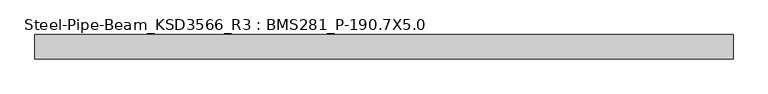
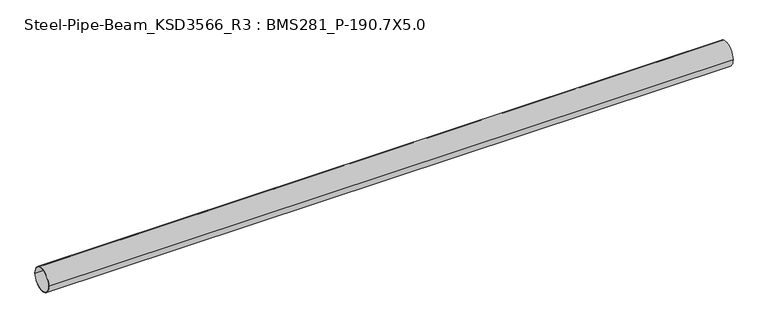
"""IFC4 building model written with IfcOpenShell, lengths in millimetres: member geometry, Steel-Pipe-Beam_KSD3566_R3 : BMS281_P-190.7X5.0."""

import ifcopenshell
import ifcopenshell.guid

model = None  # the IFC model being written
_history = None  # IfcOwnerHistory: only IFC2X3 demands one
_inside = {}  # id of a spatial element -> (the spatial element, [elements in it])
_under = {}  # id of a project, library or spatial element -> (it, [spatial elements below it])
_declared = {}  # id of a project -> (the project, [libraries it declares])
_typed = {}  # id of a type object -> (the type object, [elements of that type])
_made_of = {}  # id of a material, layer set ... -> (it, [elements and type objects made of it])


def new_model(schema):
    """Start an empty IFC model of exactly this schema.

    Asked for "IFC4X3", IfcOpenShell would pick the latest addendum, in which some entities
    have other attributes; the version numbers below select the first issue.
    IFC2X3 requires an IfcOwnerHistory on every rooted entity: one is made here for all.
    """
    global model, _history
    if schema == "IFC4X3":
        model = ifcopenshell.file(schema_version=(4, 3, 0, 0))
    else:
        model = ifcopenshell.file(schema=schema)
    _inside.clear()
    _under.clear()
    _declared.clear()
    _typed.clear()
    _made_of.clear()
    _history = None
    if model.schema == "IFC2X3":
        org = make("IfcOrganization", Name="unknown")
        user = make(
            "IfcPersonAndOrganization",
            ThePerson=make("IfcPerson", FamilyName="unknown"),
            TheOrganization=org,
        )
        app = make(
            "IfcApplication",
            ApplicationDeveloper=org,
            Version="unknown",
            ApplicationFullName="unknown",
            ApplicationIdentifier="unknown",
        )
        _history = make(
            "IfcOwnerHistory",
            OwningUser=user,
            OwningApplication=app,
            ChangeAction="ADDED",
            CreationDate=0,
        )
    return model


def make(cls, **values):
    """One entity of the class cls with the attributes given. An attribute that is None is left unset."""
    return model.create_entity(
        cls, **{name: value for name, value in values.items() if value is not None}
    )


def rooted(cls, **values):
    """An entity with a GlobalId (a new one), such as an element, a storey or a relation."""
    return make(cls, GlobalId=ifcopenshell.guid.new(), OwnerHistory=_history, **values)


def si_unit(unit_type, name, prefix=None):
    """IfcSIUnit, for example si_unit("LENGTHUNIT", "METRE", prefix="MILLI")."""
    return make("IfcSIUnit", UnitType=unit_type, Prefix=prefix, Name=name)


def assignment(units):
    """IfcUnitAssignment: the units of a project."""
    return None if units is None else make("IfcUnitAssignment", Units=units)


def point(xyz):
    """IfcCartesianPoint."""
    return None if xyz is None else make("IfcCartesianPoint", Coordinates=xyz)


def direction(xyz):
    """IfcDirection."""
    return None if xyz is None else make("IfcDirection", DirectionRatios=xyz)


def frame(location, z_axis=None, x_axis=None):
    """IfcAxis2Placement3D, a coordinate frame: its origin and axes. An axis left out is left unset."""
    return make(
        "IfcAxis2Placement3D",
        Location=point(location),
        Axis=direction(z_axis),
        RefDirection=direction(x_axis),
    )


def frame_2d(location, x_axis=None):
    """IfcAxis2Placement2D, a coordinate frame in the plane: its origin and x axis."""
    return make(
        "IfcAxis2Placement2D", Location=point(location), RefDirection=direction(x_axis)
    )


def origin():
    """The frame at (0, 0, 0) with its axes left unset."""
    return frame((0.0, 0.0, 0.0))


def origin_2d():
    """The frame at (0, 0) in the plane with its x axis left unset."""
    return frame_2d((0.0, 0.0))


def place(relative_to, where):
    """IfcLocalPlacement: puts the frame where relative to a parent placement (None: the world)."""
    return make(
        "IfcLocalPlacement", PlacementRelTo=relative_to, RelativePlacement=where
    )


def context(
    kind, dimensions, precision=None, world=None, true_north=None, identifier=None
):
    """IfcGeometricRepresentationContext, for example the 3D "Model" context."""
    return make(
        "IfcGeometricRepresentationContext",
        ContextIdentifier=identifier,
        ContextType=kind,
        CoordinateSpaceDimension=dimensions,
        Precision=precision,
        WorldCoordinateSystem=world,
        TrueNorth=true_north,
    )


def project(units=None, contexts=None):
    """IfcProject with its units and contexts."""
    return rooted(
        "IfcProject",
        Name="project",
        RepresentationContexts=contexts,
        UnitsInContext=assignment(units),
    )


def spatial(cls, under=None, at=None, **own):
    """A site, building, storey or space (cls), placed at a placement, below another one or the project."""
    s = rooted(cls, ObjectPlacement=at, **own)
    if under is not None:
        _under.setdefault(under.id(), (under, []))[1].append(s)
    return s


def circle_curve(where, radius):
    """IfcCircle in the frame where."""
    return make("IfcCircle", Position=where, Radius=radius)


def trimmed(basis, trim1, trim2, sense, master):
    """IfcTrimmedCurve: the piece of a basis curve between two trims."""
    return make(
        "IfcTrimmedCurve",
        BasisCurve=basis,
        Trim1=trim1,
        Trim2=trim2,
        SenseAgreement=sense,
        MasterRepresentation=master,
    )


def segment(curve, same_sense, transition):
    """IfcCompositeCurveSegment."""
    return make(
        "IfcCompositeCurveSegment",
        Transition=transition,
        SameSense=same_sense,
        ParentCurve=curve,
    )


def composite_curve(segments, self_intersect=None):
    """IfcCompositeCurve: segments joined end to end."""
    return make("IfcCompositeCurve", Segments=segments, SelfIntersect=self_intersect)


def outline(outer, holes=None, kind="AREA"):
    """IfcArbitraryClosedProfileDef: a profile drawn as a closed curve; with holes, ...WithVoids."""
    if holes is None:
        return make("IfcArbitraryClosedProfileDef", ProfileType=kind, OuterCurve=outer)
    return make(
        "IfcArbitraryProfileDefWithVoids",
        ProfileType=kind,
        OuterCurve=outer,
        InnerCurves=holes,
    )


def extrude(swept, where, along, depth):
    """IfcExtrudedAreaSolid: the profile swept, set in the frame where, extruded along a direction by depth."""
    return make(
        "IfcExtrudedAreaSolid",
        SweptArea=swept,
        Position=where,
        ExtrudedDirection=direction(along),
        Depth=depth,
    )


def shape(context_of_items, identifier, shape_type, items):
    """IfcShapeRepresentation: the items that make up one representation, for example the "Body"."""
    return make(
        "IfcShapeRepresentation",
        ContextOfItems=context_of_items,
        RepresentationIdentifier=identifier,
        RepresentationType=shape_type,
        Items=items,
    )


def source(mapping_origin, context_of_items, identifier, shape_type, items):
    """IfcRepresentationMap: a shape defined once, which mapped items show again and again."""
    return make(
        "IfcRepresentationMap",
        MappingOrigin=mapping_origin,
        MappedRepresentation=shape(context_of_items, identifier, shape_type, items),
    )


def transform(
    local_origin,
    x_axis=None,
    y_axis=None,
    z_axis=None,
    scale=None,
    scale2=None,
    scale3=None,
    uniform=True,
):
    """IfcCartesianTransformationOperator3D, or its non-uniform kind. x_axis, y_axis, z_axis: its Axis1, 2, 3."""
    if uniform:
        return make(
            "IfcCartesianTransformationOperator3D",
            Axis1=direction(x_axis),
            Axis2=direction(y_axis),
            LocalOrigin=point(local_origin),
            Scale=scale,
            Axis3=direction(z_axis),
        )
    return make(
        "IfcCartesianTransformationOperator3DnonUniform",
        Axis1=direction(x_axis),
        Axis2=direction(y_axis),
        LocalOrigin=point(local_origin),
        Scale=scale,
        Axis3=direction(z_axis),
        Scale2=scale2,
        Scale3=scale3,
    )


def mapped(mapping_source, mapping_target):
    """IfcMappedItem: shows the shape of a source again, moved by a transform."""
    return make(
        "IfcMappedItem", MappingSource=mapping_source, MappingTarget=mapping_target
    )


def made_of(thing, what):
    """Note that an element or type object is made of a material, layer set ...; save() writes the relation."""
    if what is not None:
        _made_of.setdefault(what.id(), (what, []))[1].append(thing)
    return thing


def element(
    cls,
    number,
    at=None,
    inside=None,
    cuts=None,
    type_object=None,
    material=None,
    context=None,
    identifier="Body",
    shape_type=None,
    held_by="IfcProductDefinitionShape",
    body=None,
    shapes=None,
    **own,
):
    """One element of the class cls, such as IfcWall. Its Tag is "e" and its number.

    at: its placement. inside: the storey or other place that contains it. cuts: it is an
    opening in that element (IfcRelVoidsElement). A single representation is given by context,
    identifier, shape_type and body (its items); several are given by shapes. held_by: the class
    of the entity that holds the representations. save() writes the other relations.
    """
    e = rooted(cls, Tag="e%d" % number, ObjectPlacement=at, **own)
    if body is not None:
        shapes = [shape(context, identifier, shape_type, body)]
    if shapes is not None:
        e.Representation = make(held_by, Representations=shapes)
    if inside is not None:
        _inside.setdefault(inside.id(), (inside, []))[1].append(e)
    if cuts is not None:
        rooted(
            "IfcRelVoidsElement", RelatingBuildingElement=cuts, RelatedOpeningElement=e
        )
    if type_object is not None:
        _typed.setdefault(type_object.id(), (type_object, []))[1].append(e)
    return made_of(e, material)


def aggregate(whole, parts):
    """IfcRelAggregates: a whole, such as a stair, and the parts it consists of."""
    return rooted("IfcRelAggregates", RelatingObject=whole, RelatedObjects=parts)


def save(model, path):
    """Write the relations noted so far, then the file.

    IfcRelAggregates (storeys below a building ...), IfcRelContainedInSpatialStructure (elements
    in a storey), IfcRelDefinesByType, IfcRelAssociatesMaterial and IfcRelDeclares: one each for
    every whole, place, type object, material and project.
    """
    for whole, parts in _under.values():
        aggregate(whole, parts)
    for where, things in _inside.values():
        rooted(
            "IfcRelContainedInSpatialStructure",
            RelatedElements=things,
            RelatingStructure=where,
        )
    for kind, things in _typed.values():
        rooted("IfcRelDefinesByType", RelatedObjects=things, RelatingType=kind)
    for what, things in _made_of.values():
        rooted("IfcRelAssociatesMaterial", RelatedObjects=things, RelatingMaterial=what)
    for by, libraries in _declared.values():
        rooted("IfcRelDeclares", RelatingContext=by, RelatedDefinitions=libraries)
    model.write(path)


def steel_pipe_beam_ksd3566_r3_bms281_p_190_7x5_0_a066e970(model_context):
    return source(origin(), model_context, "Body", "SweptSolid", [
        extrude(outline(composite_curve([segment(trimmed(circle_curve(origin_2d(), 95.35), [point((-95.35, 0.0))], [point((95.35, 0.0))], False, "CARTESIAN"), True, "CONTINUOUS"), segment(trimmed(circle_curve(origin_2d(), 95.35), [point((95.35, 0.0))], [point((-95.35, 0.0))], False, "CARTESIAN"), True, "CONTINUOUS")], self_intersect=False), holes=[composite_curve([segment(trimmed(circle_curve(origin_2d(), 90.35), [point((90.35, 0.0))], [point((-90.35, 0.0))], True, "CARTESIAN"), True, "CONTINUOUS"), segment(trimmed(circle_curve(origin_2d(), 90.35), [point((-90.35, 0.0))], [point((90.35, 0.0))], True, "CARTESIAN"), True, "CONTINUOUS")], self_intersect=False)]), frame((-2735.5137549, 0.0, 0.0), z_axis=(1.0, 0.0, 0.0), x_axis=(0.0, 1.0, 0.0)), (0.0, 0.0, 1.0), 5478.5324391),
    ])


if __name__ == "__main__":
    model = new_model("IFC4")
    model_context = context("Model", 3, world=origin())
    ifc_project = project(units=[si_unit("LENGTHUNIT", "METRE", prefix="MILLI")], contexts=[model_context])
    site = spatial("IfcSite", under=ifc_project)
    building = spatial("IfcBuilding", under=site)
    placement = place(None, origin())
    steel_pipe_beam_ksd3566_r3_bms281_p_190_7x5_0_shape = steel_pipe_beam_ksd3566_r3_bms281_p_190_7x5_0_a066e970(model_context)
    element("IfcMember", 1, ObjectType="Steel-Pipe-Beam_KSD3566_R3 : BMS281_P-190.7X5.0", at=placement, inside=building, context=model_context, shape_type="MappedRepresentation", body=[
        mapped(steel_pipe_beam_ksd3566_r3_bms281_p_190_7x5_0_shape, transform((0.0, 0.0, 0.0), x_axis=(1.0, 0.0, 0.0), y_axis=(0.0, 1.0, 0.0), z_axis=(0.0, 0.0, 1.0))),
    ])
    save(model, "model.ifc")

# Revit data of these elements
# Type "Steel-Pipe-Beam_KSD3566_R3 : BMS281_P-190.7X5.0"
#   Keynote = "P-190.7X5.0"
#   SteelWeight = "Light"
#   t = 0.0050 m
#   Surface Area = 0.599102 m²/m
#   Section Area = 29.1697 cm²
#   Mass per Unit Length = 22.8982 kg/m
#   Length [instance default] = 1.5000 m
#   D = 0.1907 m
#   hec_material4 [instance default] = none
#   hec_material3 [instance default] = none
#   hec_material2 [instance default] = none
#   hec_material1 [instance default] = none
#   Structural Material [instance default] = Steel, 45-345
#   Assembly Code = ""
# Element 1 (IfcMember, "Steel-Pipe-Beam_KSD3566_R3 : BMS281_P-190.7X5.0")
#   Structural Material = none
# Materials
#   "Steel, 45-345": class "Metal", colour RGB 189 187 185, transparency 0, Description = "Steel 345 MPa", Cost = 0
